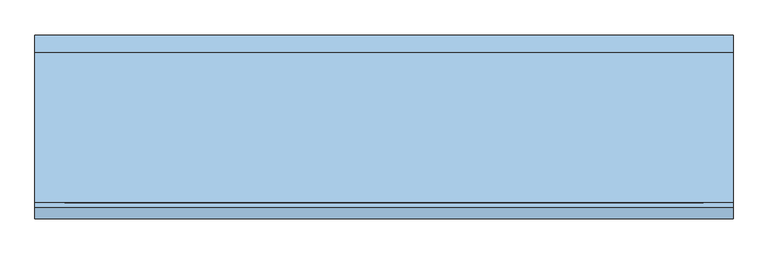
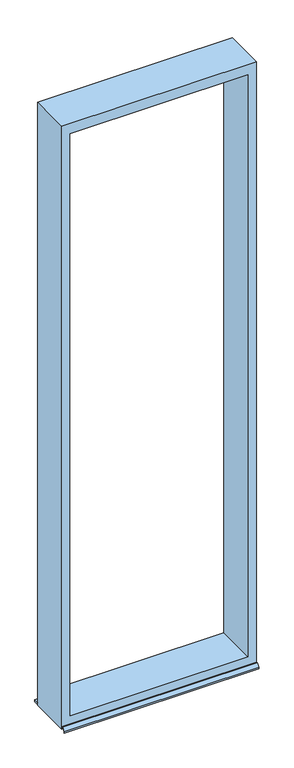
"""IFC4 building model written with IfcOpenShell, lengths in millimetres: window geometry, Fenster - Festverglasung : Feste Verglasung 4.58 x 1.40 2."""

from ifc_helpers import new_model, si_unit, frame, origin, place, context, project, spatial, polyline, outline, extrude, source, transform, mapped, element, save


def window_15a4d7c7(model_context):
    return source(origin(), model_context, "Body", "SweptSolid", [
        extrude(outline(polyline([(5580.0, 700.0), (5580.0, -700.0), (1000.0, -700.0), (1000.0, 700.0), (5580.0, 700.0)]), holes=[polyline([(5500.0, 640.0), (1080.0, 640.0), (1080.0, -640.0), (5500.0, -640.0), (5500.0, 640.0)])]), frame((0.0, -151.5214598, 0.0), z_axis=(0.0, 1.0, 0.0), x_axis=(0.0, 0.0, 1.0)), (0.0, 0.0, 1.0), 300.0),
        extrude(outline(polyline([(-700.0, 184.0), (700.0, 184.0), (700.0, 148.4785402), (-700.0, 148.4785402), (-700.0, 184.0)])), frame((0.0, 0.0, 1005.0), z_axis=(0.0, 0.0, 1.0), x_axis=(1.0, 0.0, 0.0)), (0.0, 0.0, 1.0), 15.0),
        extrude(outline(polyline([(-161.5436142, 1020.0), (-151.5214598, 1020.0), (-151.5214598, 1018.0), (-161.3455321, 1018.0), (-182.0, 998.3604634), (-182.0, 990.0), (-184.0, 990.0), (-184.0, 1000.0), (-161.5436142, 1020.0)])), frame((-700.0, 0.0, 0.0), z_axis=(1.0, 0.0, 0.0), x_axis=(0.0, 1.0, 0.0)), (0.0, 0.0, 1.0), 1400.0),
    ])


if __name__ == "__main__":
    model = new_model("IFC4")
    model_context = context("Model", 3, world=origin())
    ifc_project = project(units=[si_unit("LENGTHUNIT", "METRE", prefix="MILLI")], contexts=[model_context])
    site = spatial("IfcSite", under=ifc_project)
    building = spatial("IfcBuilding", under=site)
    placement = place(None, origin())
    window_shape = window_15a4d7c7(model_context)
    element("IfcWindow", 1, ObjectType="Fenster - Festverglasung : Feste Verglasung 4.58 x 1.40 2", at=placement, inside=building, context=model_context, shape_type="MappedRepresentation", body=[
        mapped(window_shape, transform((0.0, 0.0, 0.0), x_axis=(1.0, 0.0, 0.0), y_axis=(0.0, 1.0, 0.0), z_axis=(0.0, 0.0, 1.0))),
    ])
    save(model, "model.ifc")

# Revit data of these elements
# Type "Fenster - Festverglasung : Feste Verglasung 4.58 x 1.40 2"
#   Type Mark = "65"
#   Operation = "SinglePanel"
#   Keynote = "16.05.01"
#   Visual Light Transmittance = 0.9
#   Solar Heat Gain Coefficient = 0.78
#   Rough Width = 1.400 m
#   Rough Height = 4.580 m
#   Heat Transfer Coefficient (U) = 3.6886 W/(m²·K)
#   Rahmentiefe = 0.300 m
#   Rahmenhöhe unten = 0.080 m
#   Höhe oberer  Rahmen = 0.080 m
#   Rahmenbreite = 0.060 m
#   Height = 4.580 m
#   Einbautiefe (von außen) [instance default] = 0.080 m
#   Width = 1.400 m
#   Wall Closure = 3
#   Bild [instance default] = none
#   Glas [instance default] = none
#   Innere Fensterbank [instance default] = none
#   Äußere Fensterbank [instance default] = none
#   Construction Type Id = ""
#   Analytic Construction = (empty or 0)
# Element 1 (IfcWindow, "Fenster - Festverglasung : Feste Verglasung 4.58 x 1.40 2")
#   Einbautiefe (von außen) = 0.002479 m
#   Materials on its faces: "Kunststoff - Weiß", "Holz - Birke"
# Materials
#   "Kunststoff - Weiß": class "Kunststoff", colour RGB 249 249 249, transparency 0, Cost = 0
#   "Holz - Birke": class "Holz", colour RGB 213 164 103, transparency 0, Cost = 0
